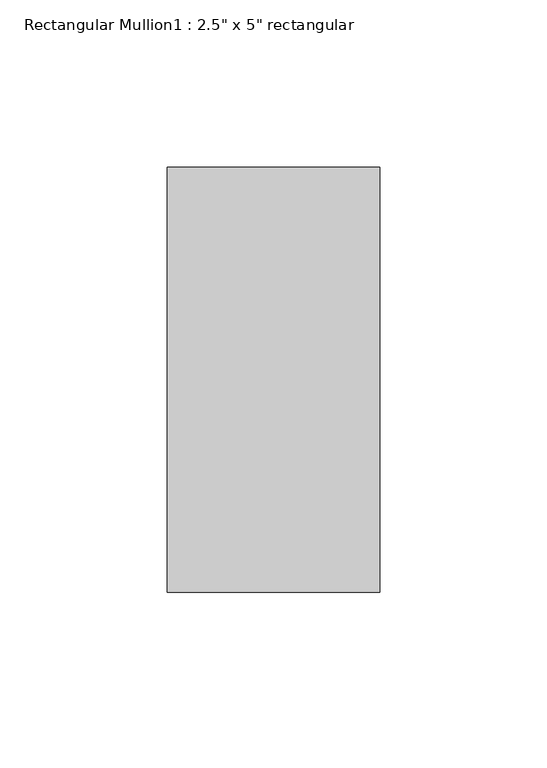
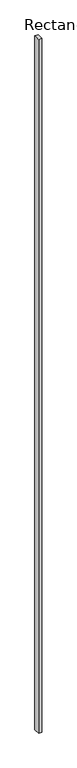
"""IFC4 building model written with IfcOpenShell, lengths in millimetres: member geometry."""

from ifc_helpers import new_model, si_unit, frame, origin, place, context, project, spatial, polyline, outline, extrude, source, transform, mapped, element, save


def member_8669c44b(model_context):
    return source(origin(), model_context, "Body", "SweptSolid", [
        extrude(outline(polyline([(31.75, 63.5), (31.75, -63.5), (-31.75, -63.5), (-31.75, 63.5), (31.75, 63.5)])), frame((0.0, 0.0, -14960.6), z_axis=(0.0, 0.0, 1.0), x_axis=(1.0, 0.0, 0.0)), (0.0, 0.0, 1.0), 14960.6),
    ])


if __name__ == "__main__":
    model = new_model("IFC4")
    model_context = context("Model", 3, world=origin())
    ifc_project = project(units=[si_unit("LENGTHUNIT", "METRE", prefix="MILLI")], contexts=[model_context])
    site = spatial("IfcSite", under=ifc_project)
    building = spatial("IfcBuilding", under=site)
    placement = place(None, origin())
    member_shape = member_8669c44b(model_context)
    element("IfcMember", 1, ObjectType="Rectangular Mullion1 : 2.5\" x 5\" rectangular", at=placement, inside=building, context=model_context, shape_type="MappedRepresentation", body=[
        mapped(member_shape, transform((0.0, 0.0, 0.0), x_axis=(1.0, 0.0, 0.0), y_axis=(0.0, 1.0, 0.0), z_axis=(0.0, 0.0, 1.0))),
    ])
    save(model, "model.ifc")

# Revit data of these elements
# Type "Rectangular Mullion1 : 2.5\" x 5\" rectangular"
#   built-in parameter 1007304 = 0.416667 (stored number, unit not read)
#   built-in parameter 1007301 = 0.104167 (stored number, unit not read)
#   built-in parameter 1007300 = 0.104167 (stored number, unit not read)
# Element 1 (IfcMember, "Rectangular Mullion1 : 2.5\" x 5\" rectangular")
#   Materials on its faces: "support-frame"
# Materials
#   "support-frame": class "Unassigned", colour RGB 233 233 233, transparency 0, Cost = 0
